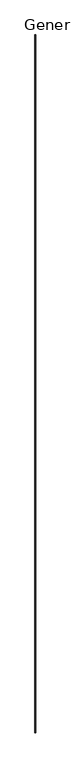
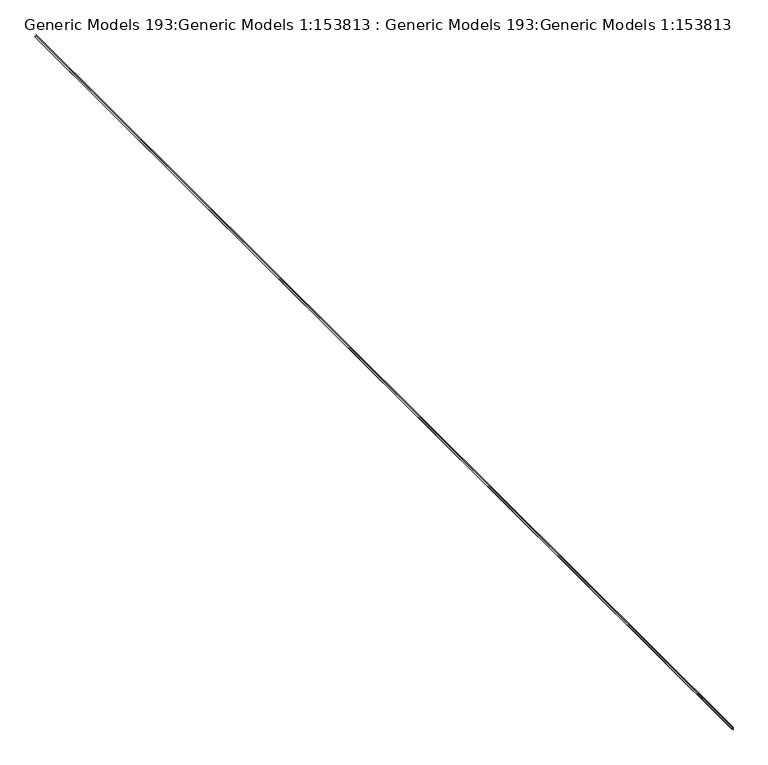
"""IFC4 building model written with IfcOpenShell, lengths in millimetres: proxy geometry, Generic Models 193:Generic Models 1:153813 : Generic Models 193:Generic Models 1:153813."""

from ifc_helpers import new_model, si_unit, frame, origin, place, context, project, spatial, polyline, outline, extrude, source, transform, mapped, element, save


def generic_models_193_generic_models_1_153813_generic_models_53e0fe61(model_context):
    return source(origin(), model_context, "Body", "SweptSolid", [
        extrude(outline(polyline([(6040.832074, -5374.8543913), (6080.202074, -5374.8543913), (6080.202074, -5376.1243913), (6061.152074, -5376.1243913), (6061.152074, -5397.0793913), (6056.402274, -5397.0793913), (6056.402274, -5395.8093913), (6059.882074, -5395.8093913), (6059.882074, -5376.1243913), (6040.832074, -5376.1243913), (6040.832074, -5374.8543913)])), frame((0.0, -6877.9974793, 0.0), z_axis=(0.0, 1.0, 0.0), x_axis=(0.0, 0.0, 1.0)), (0.0, 0.0, 1.0), 19050.0),
    ])


if __name__ == "__main__":
    model = new_model("IFC4")
    model_context = context("Model", 3, world=origin())
    ifc_project = project(units=[si_unit("LENGTHUNIT", "METRE", prefix="MILLI")], contexts=[model_context])
    site = spatial("IfcSite", under=ifc_project)
    building = spatial("IfcBuilding", under=site)
    placement = place(None, origin())
    generic_models_193_generic_models_1_153813_generic_models_shape = generic_models_193_generic_models_1_153813_generic_models_53e0fe61(model_context)
    element("IfcBuildingElementProxy", 1, Name="Generic Models 193:Generic Models 1:153813 : Generic Models 193:Generic Models 1:153813", ObjectType="Generic Models 193:Generic Models 1:153813 : Generic Models 193:Generic Models 1:153813", at=placement, inside=building, context=model_context, shape_type="MappedRepresentation", body=[
        mapped(generic_models_193_generic_models_1_153813_generic_models_shape, transform((0.0, 0.0, 0.0), x_axis=(1.0, 0.0, 0.0), y_axis=(0.0, 1.0, 0.0), z_axis=(0.0, 0.0, 1.0))),
    ])
    save(model, "model.ifc")

# Revit data of these elements
# Type "Generic Models 193:Generic Models 1:153813 : Generic Models 193:Generic Models 1:153813"
#   NameOverride = "Generic Models 193:Generic Models 1:153813"
#   ObjectTypeOverride = "Generic Models 193:Generic Models 1"
#   Reference = "Generic Models 1"
#   Category = "Generic Models"
#   Tag = "153813"
# Element 1 (IfcBuildingElementProxy, "Generic Models 193:Generic Models 1:153813 : Generic Models 193:Generic Models 1:153813")
#   Materials on its faces: "_ 16 GA. COPPER VENTED T REVEAL BEAD (CONT. AROUND PERIMETER OF BEAM) 2987"
# Materials
#   "_ 16 GA. COPPER VENTED T REVEAL BEAD (CONT. AROUND PERIMETER OF BEAM) 2987": class "Unassigned", colour RGB 253 192 103, transparency 0
